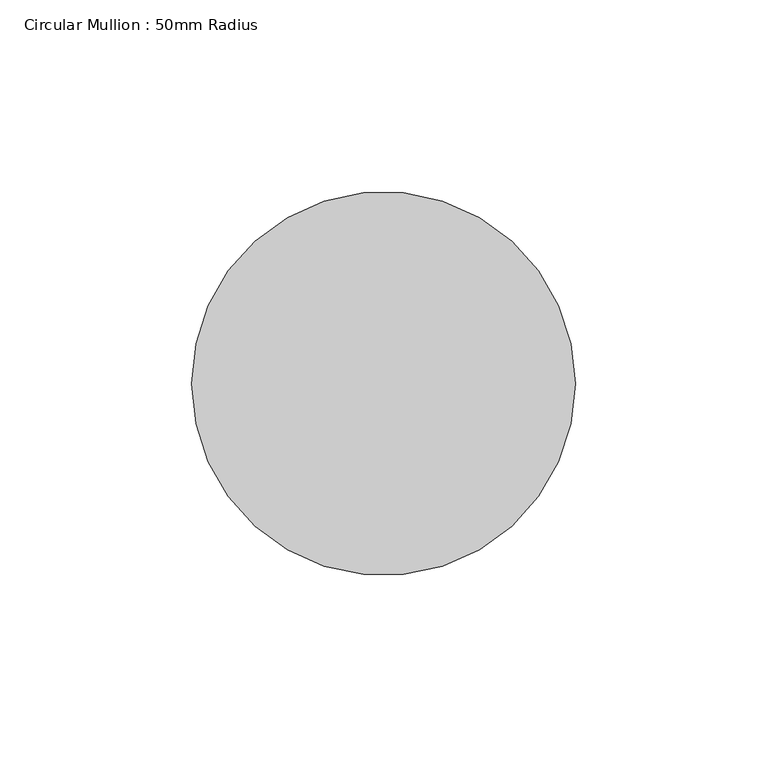
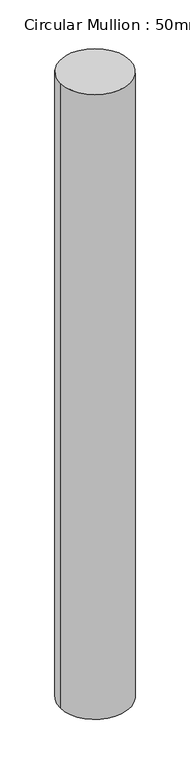
"""IFC4 building model written with IfcOpenShell, lengths in millimetres: member geometry, Circular Mullion : 50mm Radius."""

import ifcopenshell
import ifcopenshell.guid

model = None  # the IFC model being written
_history = None  # IfcOwnerHistory: only IFC2X3 demands one
_inside = {}  # id of a spatial element -> (the spatial element, [elements in it])
_under = {}  # id of a project, library or spatial element -> (it, [spatial elements below it])
_declared = {}  # id of a project -> (the project, [libraries it declares])
_typed = {}  # id of a type object -> (the type object, [elements of that type])
_made_of = {}  # id of a material, layer set ... -> (it, [elements and type objects made of it])


def new_model(schema):
    """Start an empty IFC model of exactly this schema.

    Asked for "IFC4X3", IfcOpenShell would pick the latest addendum, in which some entities
    have other attributes; the version numbers below select the first issue.
    IFC2X3 requires an IfcOwnerHistory on every rooted entity: one is made here for all.
    """
    global model, _history
    if schema == "IFC4X3":
        model = ifcopenshell.file(schema_version=(4, 3, 0, 0))
    else:
        model = ifcopenshell.file(schema=schema)
    _inside.clear()
    _under.clear()
    _declared.clear()
    _typed.clear()
    _made_of.clear()
    _history = None
    if model.schema == "IFC2X3":
        org = make("IfcOrganization", Name="unknown")
        user = make(
            "IfcPersonAndOrganization",
            ThePerson=make("IfcPerson", FamilyName="unknown"),
            TheOrganization=org,
        )
        app = make(
            "IfcApplication",
            ApplicationDeveloper=org,
            Version="unknown",
            ApplicationFullName="unknown",
            ApplicationIdentifier="unknown",
        )
        _history = make(
            "IfcOwnerHistory",
            OwningUser=user,
            OwningApplication=app,
            ChangeAction="ADDED",
            CreationDate=0,
        )
    return model


def make(cls, **values):
    """One entity of the class cls with the attributes given. An attribute that is None is left unset."""
    return model.create_entity(
        cls, **{name: value for name, value in values.items() if value is not None}
    )


def rooted(cls, **values):
    """An entity with a GlobalId (a new one), such as an element, a storey or a relation."""
    return make(cls, GlobalId=ifcopenshell.guid.new(), OwnerHistory=_history, **values)


def si_unit(unit_type, name, prefix=None):
    """IfcSIUnit, for example si_unit("LENGTHUNIT", "METRE", prefix="MILLI")."""
    return make("IfcSIUnit", UnitType=unit_type, Prefix=prefix, Name=name)


def assignment(units):
    """IfcUnitAssignment: the units of a project."""
    return None if units is None else make("IfcUnitAssignment", Units=units)


def point(xyz):
    """IfcCartesianPoint."""
    return None if xyz is None else make("IfcCartesianPoint", Coordinates=xyz)


def direction(xyz):
    """IfcDirection."""
    return None if xyz is None else make("IfcDirection", DirectionRatios=xyz)


def frame(location, z_axis=None, x_axis=None):
    """IfcAxis2Placement3D, a coordinate frame: its origin and axes. An axis left out is left unset."""
    return make(
        "IfcAxis2Placement3D",
        Location=point(location),
        Axis=direction(z_axis),
        RefDirection=direction(x_axis),
    )


def frame_2d(location, x_axis=None):
    """IfcAxis2Placement2D, a coordinate frame in the plane: its origin and x axis."""
    return make(
        "IfcAxis2Placement2D", Location=point(location), RefDirection=direction(x_axis)
    )


def origin():
    """The frame at (0, 0, 0) with its axes left unset."""
    return frame((0.0, 0.0, 0.0))


def origin_2d():
    """The frame at (0, 0) in the plane with its x axis left unset."""
    return frame_2d((0.0, 0.0))


def place(relative_to, where):
    """IfcLocalPlacement: puts the frame where relative to a parent placement (None: the world)."""
    return make(
        "IfcLocalPlacement", PlacementRelTo=relative_to, RelativePlacement=where
    )


def context(
    kind, dimensions, precision=None, world=None, true_north=None, identifier=None
):
    """IfcGeometricRepresentationContext, for example the 3D "Model" context."""
    return make(
        "IfcGeometricRepresentationContext",
        ContextIdentifier=identifier,
        ContextType=kind,
        CoordinateSpaceDimension=dimensions,
        Precision=precision,
        WorldCoordinateSystem=world,
        TrueNorth=true_north,
    )


def project(units=None, contexts=None):
    """IfcProject with its units and contexts."""
    return rooted(
        "IfcProject",
        Name="project",
        RepresentationContexts=contexts,
        UnitsInContext=assignment(units),
    )


def spatial(cls, under=None, at=None, **own):
    """A site, building, storey or space (cls), placed at a placement, below another one or the project."""
    s = rooted(cls, ObjectPlacement=at, **own)
    if under is not None:
        _under.setdefault(under.id(), (under, []))[1].append(s)
    return s


def circle_curve(where, radius):
    """IfcCircle in the frame where."""
    return make("IfcCircle", Position=where, Radius=radius)


def trimmed(basis, trim1, trim2, sense, master):
    """IfcTrimmedCurve: the piece of a basis curve between two trims."""
    return make(
        "IfcTrimmedCurve",
        BasisCurve=basis,
        Trim1=trim1,
        Trim2=trim2,
        SenseAgreement=sense,
        MasterRepresentation=master,
    )


def segment(curve, same_sense, transition):
    """IfcCompositeCurveSegment."""
    return make(
        "IfcCompositeCurveSegment",
        Transition=transition,
        SameSense=same_sense,
        ParentCurve=curve,
    )


def composite_curve(segments, self_intersect=None):
    """IfcCompositeCurve: segments joined end to end."""
    return make("IfcCompositeCurve", Segments=segments, SelfIntersect=self_intersect)


def outline(outer, holes=None, kind="AREA"):
    """IfcArbitraryClosedProfileDef: a profile drawn as a closed curve; with holes, ...WithVoids."""
    if holes is None:
        return make("IfcArbitraryClosedProfileDef", ProfileType=kind, OuterCurve=outer)
    return make(
        "IfcArbitraryProfileDefWithVoids",
        ProfileType=kind,
        OuterCurve=outer,
        InnerCurves=holes,
    )


def extrude(swept, where, along, depth):
    """IfcExtrudedAreaSolid: the profile swept, set in the frame where, extruded along a direction by depth."""
    return make(
        "IfcExtrudedAreaSolid",
        SweptArea=swept,
        Position=where,
        ExtrudedDirection=direction(along),
        Depth=depth,
    )


def shape(context_of_items, identifier, shape_type, items):
    """IfcShapeRepresentation: the items that make up one representation, for example the "Body"."""
    return make(
        "IfcShapeRepresentation",
        ContextOfItems=context_of_items,
        RepresentationIdentifier=identifier,
        RepresentationType=shape_type,
        Items=items,
    )


def source(mapping_origin, context_of_items, identifier, shape_type, items):
    """IfcRepresentationMap: a shape defined once, which mapped items show again and again."""
    return make(
        "IfcRepresentationMap",
        MappingOrigin=mapping_origin,
        MappedRepresentation=shape(context_of_items, identifier, shape_type, items),
    )


def transform(
    local_origin,
    x_axis=None,
    y_axis=None,
    z_axis=None,
    scale=None,
    scale2=None,
    scale3=None,
    uniform=True,
):
    """IfcCartesianTransformationOperator3D, or its non-uniform kind. x_axis, y_axis, z_axis: its Axis1, 2, 3."""
    if uniform:
        return make(
            "IfcCartesianTransformationOperator3D",
            Axis1=direction(x_axis),
            Axis2=direction(y_axis),
            LocalOrigin=point(local_origin),
            Scale=scale,
            Axis3=direction(z_axis),
        )
    return make(
        "IfcCartesianTransformationOperator3DnonUniform",
        Axis1=direction(x_axis),
        Axis2=direction(y_axis),
        LocalOrigin=point(local_origin),
        Scale=scale,
        Axis3=direction(z_axis),
        Scale2=scale2,
        Scale3=scale3,
    )


def mapped(mapping_source, mapping_target):
    """IfcMappedItem: shows the shape of a source again, moved by a transform."""
    return make(
        "IfcMappedItem", MappingSource=mapping_source, MappingTarget=mapping_target
    )


def made_of(thing, what):
    """Note that an element or type object is made of a material, layer set ...; save() writes the relation."""
    if what is not None:
        _made_of.setdefault(what.id(), (what, []))[1].append(thing)
    return thing


def element(
    cls,
    number,
    at=None,
    inside=None,
    cuts=None,
    type_object=None,
    material=None,
    context=None,
    identifier="Body",
    shape_type=None,
    held_by="IfcProductDefinitionShape",
    body=None,
    shapes=None,
    **own,
):
    """One element of the class cls, such as IfcWall. Its Tag is "e" and its number.

    at: its placement. inside: the storey or other place that contains it. cuts: it is an
    opening in that element (IfcRelVoidsElement). A single representation is given by context,
    identifier, shape_type and body (its items); several are given by shapes. held_by: the class
    of the entity that holds the representations. save() writes the other relations.
    """
    e = rooted(cls, Tag="e%d" % number, ObjectPlacement=at, **own)
    if body is not None:
        shapes = [shape(context, identifier, shape_type, body)]
    if shapes is not None:
        e.Representation = make(held_by, Representations=shapes)
    if inside is not None:
        _inside.setdefault(inside.id(), (inside, []))[1].append(e)
    if cuts is not None:
        rooted(
            "IfcRelVoidsElement", RelatingBuildingElement=cuts, RelatedOpeningElement=e
        )
    if type_object is not None:
        _typed.setdefault(type_object.id(), (type_object, []))[1].append(e)
    return made_of(e, material)


def aggregate(whole, parts):
    """IfcRelAggregates: a whole, such as a stair, and the parts it consists of."""
    return rooted("IfcRelAggregates", RelatingObject=whole, RelatedObjects=parts)


def save(model, path):
    """Write the relations noted so far, then the file.

    IfcRelAggregates (storeys below a building ...), IfcRelContainedInSpatialStructure (elements
    in a storey), IfcRelDefinesByType, IfcRelAssociatesMaterial and IfcRelDeclares: one each for
    every whole, place, type object, material and project.
    """
    for whole, parts in _under.values():
        aggregate(whole, parts)
    for where, things in _inside.values():
        rooted(
            "IfcRelContainedInSpatialStructure",
            RelatedElements=things,
            RelatingStructure=where,
        )
    for kind, things in _typed.values():
        rooted("IfcRelDefinesByType", RelatedObjects=things, RelatingType=kind)
    for what, things in _made_of.values():
        rooted("IfcRelAssociatesMaterial", RelatedObjects=things, RelatingMaterial=what)
    for by, libraries in _declared.values():
        rooted("IfcRelDeclares", RelatingContext=by, RelatedDefinitions=libraries)
    model.write(path)


def circular_mullion_50mm_radius_ce6a5862(model_context):
    return source(origin(), model_context, "Body", "SweptSolid", [
        extrude(outline(composite_curve([segment(trimmed(circle_curve(origin_2d(), 50.0), [point((50.0, 0.0))], [point((-50.0, 0.0))], False, "CARTESIAN"), True, "CONTINUOUS"), segment(trimmed(circle_curve(origin_2d(), 50.0), [point((-50.0, 0.0))], [point((50.0, 0.0))], False, "CARTESIAN"), True, "CONTINUOUS")], self_intersect=False)), frame((0.0, 0.0, -949.8832332), z_axis=(0.0, 0.0, 1.0), x_axis=(1.0, 0.0, 0.0)), (0.0, 0.0, 1.0), 949.8832332),
    ])


if __name__ == "__main__":
    model = new_model("IFC4")
    model_context = context("Model", 3, world=origin())
    ifc_project = project(units=[si_unit("LENGTHUNIT", "METRE", prefix="MILLI")], contexts=[model_context])
    site = spatial("IfcSite", under=ifc_project)
    building = spatial("IfcBuilding", under=site)
    placement = place(None, origin())
    circular_mullion_50mm_radius_shape = circular_mullion_50mm_radius_ce6a5862(model_context)
    element("IfcMember", 1, ObjectType="Circular Mullion : 50mm Radius", at=placement, inside=building, context=model_context, shape_type="MappedRepresentation", body=[
        mapped(circular_mullion_50mm_radius_shape, transform((0.0, 0.0, 0.0), x_axis=(1.0, 0.0, 0.0), y_axis=(0.0, 1.0, 0.0), z_axis=(0.0, 0.0, 1.0))),
    ])
    save(model, "model.ifc")

# Revit data of these elements
# Type "Circular Mullion : 50mm Radius"
#   built-in parameter 1007350 = 0.164042 (stored number, unit not read)
# Element 1 (IfcMember, "Circular Mullion : 50mm Radius")
#   Materials on its faces: "Aluminium"
# Materials
#   "Aluminium": class "Metal", colour RGB 247 247 247, transparency 0, Description = "Aluminium 6061", Cost = 0
